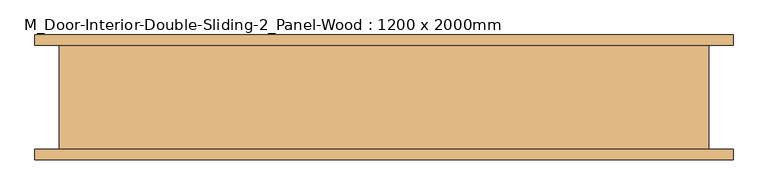
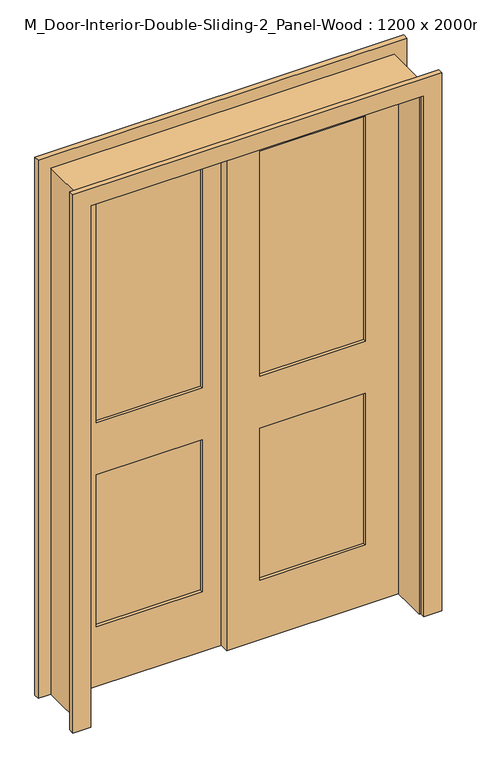
"""IFC4 building model written with IfcOpenShell, lengths in millimetres: door geometry, M_Door-Interior-Double-Sliding-2_Panel-Wood : 1200 x 2000mm."""

from ifc_helpers import new_model, si_unit, frame, origin, place, context, project, spatial, polyline, outline, extrude, source, transform, mapped, element, save


def m_door_interior_double_sliding_2_panel_wood_1200_x_2000mm_2523b4d6(model_context):
    return source(origin(), model_context, "Body", "SweptSolid", [
        extrude(outline(polyline([(480.0, 38.4916667), (94.6, 38.4916667), (94.6, 50.1583333), (480.0, 50.1583333), (480.0, 38.4916667)])), frame((0.0, 0.0, 1014.4), z_axis=(0.0, 0.0, 1.0), x_axis=(1.0, 0.0, 0.0)), (0.0, 0.0, 1.0), 865.6),
        extrude(outline(polyline([(480.0, 38.4916667), (94.6, 38.4916667), (94.6, 50.1583333), (480.0, 50.1583333), (480.0, 38.4916667)])), frame((0.0, 0.0, 230.0), z_axis=(0.0, 0.0, 1.0), x_axis=(1.0, 0.0, 0.0)), (0.0, 0.0, 1.0), 584.4),
        extrude(outline(polyline([(2000.0, -25.4), (0.0, -25.4), (0.0, 600.0), (2000.0, 600.0), (2000.0, -25.4)]), holes=[polyline([(1880.0, 94.6), (1880.0, 480.0), (1014.4, 480.0), (1014.4, 94.6), (1880.0, 94.6)]), polyline([(814.4, 94.6), (814.4, 480.0), (230.0, 480.0), (230.0, 94.6), (814.4, 94.6)])]), frame((0.0, 26.825, 0.0), z_axis=(0.0, 1.0, 0.0), x_axis=(0.0, 0.0, 1.0)), (0.0, 0.0, 1.0), 35.0),
        extrude(outline(polyline([(-94.6, 73.4916667), (-480.0, 73.4916667), (-480.0, 85.1583333), (-94.6, 85.1583333), (-94.6, 73.4916667)])), frame((0.0, 0.0, 1014.4), z_axis=(0.0, 0.0, 1.0), x_axis=(1.0, 0.0, 0.0)), (0.0, 0.0, 1.0), 865.6),
        extrude(outline(polyline([(-94.6, 73.4916667), (-480.0, 73.4916667), (-480.0, 85.1583333), (-94.6, 85.1583333), (-94.6, 73.4916667)])), frame((0.0, 0.0, 230.0), z_axis=(0.0, 0.0, 1.0), x_axis=(1.0, 0.0, 0.0)), (0.0, 0.0, 1.0), 584.4),
        extrude(outline(polyline([(2000.0, -600.0), (0.0, -600.0), (0.0, 25.4), (2000.0, 25.4), (2000.0, -600.0)]), holes=[polyline([(1880.0, -480.0), (1880.0, -94.6), (1014.4, -94.6), (1014.4, -480.0), (1880.0, -480.0)]), polyline([(814.4, -480.0), (814.4, -94.6), (230.0, -94.6), (230.0, -480.0), (814.4, -480.0)])]), frame((0.0, 61.825, 0.0), z_axis=(0.0, 1.0, 0.0), x_axis=(0.0, 0.0, 1.0)), (0.0, 0.0, 1.0), 35.0),
        extrude(outline(polyline([(0.0, 600.0), (0.0, 625.0), (2025.0, 625.0), (2025.0, -625.0), (0.0, -625.0), (0.0, -600.0), (2000.0, -600.0), (2000.0, 600.0), (0.0, 600.0)])), frame((0.0, -103.175, 0.0), z_axis=(0.0, 1.0, 0.0), x_axis=(0.0, 0.0, 1.0)), (0.0, 0.0, 1.0), 200.0),
        extrude(outline(polyline([(0.0, 606.35), (0.0, 671.35), (2071.35, 671.35), (2071.35, -671.35), (0.0, -671.35), (0.0, -606.35), (2006.35, -606.35), (2006.35, 606.35), (0.0, 606.35)])), frame((0.0, -123.175, 0.0), z_axis=(0.0, 1.0, 0.0), x_axis=(0.0, 0.0, 1.0)), (0.0, 0.0, 1.0), 20.0),
        extrude(outline(polyline([(0.0, 606.35), (0.0, 671.35), (2071.35, 671.35), (2071.35, -671.35), (0.0, -671.35), (0.0, -606.35), (2006.35, -606.35), (2006.35, 606.35), (0.0, 606.35)])), frame((0.0, 96.825, 0.0), z_axis=(0.0, 1.0, 0.0), x_axis=(0.0, 0.0, 1.0)), (0.0, 0.0, 1.0), 20.0),
    ])


if __name__ == "__main__":
    model = new_model("IFC4")
    model_context = context("Model", 3, world=origin())
    ifc_project = project(units=[si_unit("LENGTHUNIT", "METRE", prefix="MILLI")], contexts=[model_context])
    site = spatial("IfcSite", under=ifc_project)
    building = spatial("IfcBuilding", under=site)
    placement = place(None, origin())
    m_door_interior_double_sliding_2_panel_wood_1200_x_2000mm_shape = m_door_interior_double_sliding_2_panel_wood_1200_x_2000mm_2523b4d6(model_context)
    element("IfcDoor", 1, ObjectType="M_Door-Interior-Double-Sliding-2_Panel-Wood : 1200 x 2000mm", at=placement, inside=building, context=model_context, shape_type="MappedRepresentation", body=[
        mapped(m_door_interior_double_sliding_2_panel_wood_1200_x_2000mm_shape, transform((0.0, 0.0, 0.0), x_axis=(1.0, 0.0, 0.0), y_axis=(0.0, 1.0, 0.0), z_axis=(0.0, 0.0, 1.0))),
    ])
    save(model, "model.ifc")

# Revit data of these elements
# Type "M_Door-Interior-Double-Sliding-2_Panel-Wood : 1200 x 2000mm"
#   Type Mark = "23"
#   Assembly Code = "C1020300"
#   Analytic Construction = "Wooden"
#   Top Rail = 0' - 4.72441"
#   Thickness = 0' - 1.37795"
#   Thermal Resistance (R) = 0.455703 (m²·K)/W
#   Stiles = 0' - 4.72441"
#   Rough Width = 4' - 1.2126"
#   Rough Height = 6' - 7.72441"
#   Lock Rail = 0' - 7.87402"
#   Height = 6' - 6.74016"
#   Width = 3' - 11.24409"
#   Heat Transfer Coefficient (U) = 2.19465 W/(m²·K)
#   Bottom Rail = 0' - 9.05512"
#   Trim Material = Cherry
#   Panel Material = Cherry
#   Frame Material = Cherry
#   Visual Light Transmittance = 0
#   Solar Heat Gain Coefficient = 0
#   Wall Closure = (empty or 0)
#   Function = (empty or 0)
# Element 1 (IfcDoor, "M_Door-Interior-Double-Sliding-2_Panel-Wood : 1200 x 2000mm")
#   Materials on its faces: "Cherry"
# Materials
#   "Cherry": class "Wood", colour RGB 226 177 128, transparency 0, Description = "Prunus Serotina", Cost = 0
